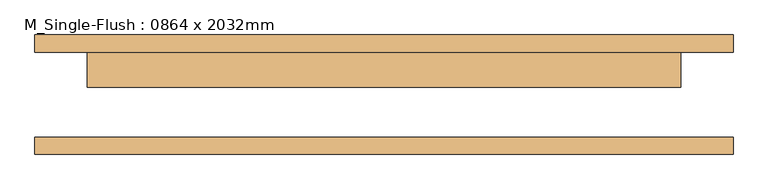
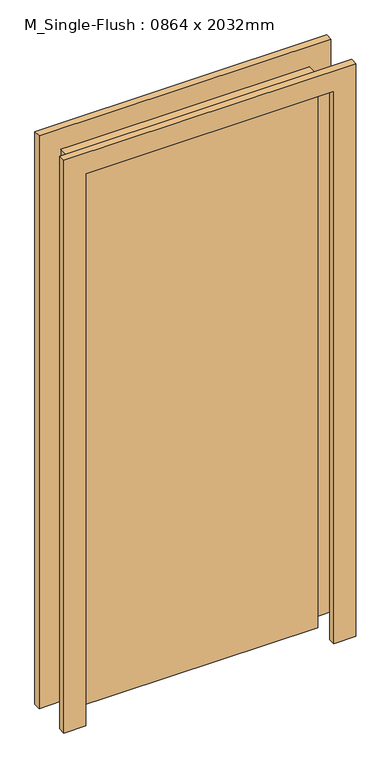
"""IFC4 building model written with IfcOpenShell, lengths in millimetres: door geometry, M_Single-Flush : 0864 x 2032mm."""

import ifcopenshell
import ifcopenshell.guid

model = None  # the IFC model being written
_history = None  # IfcOwnerHistory: only IFC2X3 demands one
_inside = {}  # id of a spatial element -> (the spatial element, [elements in it])
_under = {}  # id of a project, library or spatial element -> (it, [spatial elements below it])
_declared = {}  # id of a project -> (the project, [libraries it declares])
_typed = {}  # id of a type object -> (the type object, [elements of that type])
_made_of = {}  # id of a material, layer set ... -> (it, [elements and type objects made of it])


def new_model(schema):
    """Start an empty IFC model of exactly this schema.

    Asked for "IFC4X3", IfcOpenShell would pick the latest addendum, in which some entities
    have other attributes; the version numbers below select the first issue.
    IFC2X3 requires an IfcOwnerHistory on every rooted entity: one is made here for all.
    """
    global model, _history
    if schema == "IFC4X3":
        model = ifcopenshell.file(schema_version=(4, 3, 0, 0))
    else:
        model = ifcopenshell.file(schema=schema)
    _inside.clear()
    _under.clear()
    _declared.clear()
    _typed.clear()
    _made_of.clear()
    _history = None
    if model.schema == "IFC2X3":
        org = make("IfcOrganization", Name="unknown")
        user = make(
            "IfcPersonAndOrganization",
            ThePerson=make("IfcPerson", FamilyName="unknown"),
            TheOrganization=org,
        )
        app = make(
            "IfcApplication",
            ApplicationDeveloper=org,
            Version="unknown",
            ApplicationFullName="unknown",
            ApplicationIdentifier="unknown",
        )
        _history = make(
            "IfcOwnerHistory",
            OwningUser=user,
            OwningApplication=app,
            ChangeAction="ADDED",
            CreationDate=0,
        )
    return model


def make(cls, **values):
    """One entity of the class cls with the attributes given. An attribute that is None is left unset."""
    return model.create_entity(
        cls, **{name: value for name, value in values.items() if value is not None}
    )


def rooted(cls, **values):
    """An entity with a GlobalId (a new one), such as an element, a storey or a relation."""
    return make(cls, GlobalId=ifcopenshell.guid.new(), OwnerHistory=_history, **values)


def si_unit(unit_type, name, prefix=None):
    """IfcSIUnit, for example si_unit("LENGTHUNIT", "METRE", prefix="MILLI")."""
    return make("IfcSIUnit", UnitType=unit_type, Prefix=prefix, Name=name)


def assignment(units):
    """IfcUnitAssignment: the units of a project."""
    return None if units is None else make("IfcUnitAssignment", Units=units)


def point(xyz):
    """IfcCartesianPoint."""
    return None if xyz is None else make("IfcCartesianPoint", Coordinates=xyz)


def direction(xyz):
    """IfcDirection."""
    return None if xyz is None else make("IfcDirection", DirectionRatios=xyz)


def frame(location, z_axis=None, x_axis=None):
    """IfcAxis2Placement3D, a coordinate frame: its origin and axes. An axis left out is left unset."""
    return make(
        "IfcAxis2Placement3D",
        Location=point(location),
        Axis=direction(z_axis),
        RefDirection=direction(x_axis),
    )


def origin():
    """The frame at (0, 0, 0) with its axes left unset."""
    return frame((0.0, 0.0, 0.0))


def origin_with_axes():
    """The frame at (0, 0, 0) with the z axis (0, 0, 1) and the x axis (1, 0, 0) written out."""
    return frame((0.0, 0.0, 0.0), z_axis=(0.0, 0.0, 1.0), x_axis=(1.0, 0.0, 0.0))


def place(relative_to, where):
    """IfcLocalPlacement: puts the frame where relative to a parent placement (None: the world)."""
    return make(
        "IfcLocalPlacement", PlacementRelTo=relative_to, RelativePlacement=where
    )


def context(
    kind, dimensions, precision=None, world=None, true_north=None, identifier=None
):
    """IfcGeometricRepresentationContext, for example the 3D "Model" context."""
    return make(
        "IfcGeometricRepresentationContext",
        ContextIdentifier=identifier,
        ContextType=kind,
        CoordinateSpaceDimension=dimensions,
        Precision=precision,
        WorldCoordinateSystem=world,
        TrueNorth=true_north,
    )


def project(units=None, contexts=None):
    """IfcProject with its units and contexts."""
    return rooted(
        "IfcProject",
        Name="project",
        RepresentationContexts=contexts,
        UnitsInContext=assignment(units),
    )


def spatial(cls, under=None, at=None, **own):
    """A site, building, storey or space (cls), placed at a placement, below another one or the project."""
    s = rooted(cls, ObjectPlacement=at, **own)
    if under is not None:
        _under.setdefault(under.id(), (under, []))[1].append(s)
    return s


def polyline(points):
    """IfcPolyline through the points."""
    return make("IfcPolyline", Points=[point(p) for p in points])


def outline(outer, holes=None, kind="AREA"):
    """IfcArbitraryClosedProfileDef: a profile drawn as a closed curve; with holes, ...WithVoids."""
    if holes is None:
        return make("IfcArbitraryClosedProfileDef", ProfileType=kind, OuterCurve=outer)
    return make(
        "IfcArbitraryProfileDefWithVoids",
        ProfileType=kind,
        OuterCurve=outer,
        InnerCurves=holes,
    )


def extrude(swept, where, along, depth):
    """IfcExtrudedAreaSolid: the profile swept, set in the frame where, extruded along a direction by depth."""
    return make(
        "IfcExtrudedAreaSolid",
        SweptArea=swept,
        Position=where,
        ExtrudedDirection=direction(along),
        Depth=depth,
    )


def shape(context_of_items, identifier, shape_type, items):
    """IfcShapeRepresentation: the items that make up one representation, for example the "Body"."""
    return make(
        "IfcShapeRepresentation",
        ContextOfItems=context_of_items,
        RepresentationIdentifier=identifier,
        RepresentationType=shape_type,
        Items=items,
    )


def source(mapping_origin, context_of_items, identifier, shape_type, items):
    """IfcRepresentationMap: a shape defined once, which mapped items show again and again."""
    return make(
        "IfcRepresentationMap",
        MappingOrigin=mapping_origin,
        MappedRepresentation=shape(context_of_items, identifier, shape_type, items),
    )


def transform(
    local_origin,
    x_axis=None,
    y_axis=None,
    z_axis=None,
    scale=None,
    scale2=None,
    scale3=None,
    uniform=True,
):
    """IfcCartesianTransformationOperator3D, or its non-uniform kind. x_axis, y_axis, z_axis: its Axis1, 2, 3."""
    if uniform:
        return make(
            "IfcCartesianTransformationOperator3D",
            Axis1=direction(x_axis),
            Axis2=direction(y_axis),
            LocalOrigin=point(local_origin),
            Scale=scale,
            Axis3=direction(z_axis),
        )
    return make(
        "IfcCartesianTransformationOperator3DnonUniform",
        Axis1=direction(x_axis),
        Axis2=direction(y_axis),
        LocalOrigin=point(local_origin),
        Scale=scale,
        Axis3=direction(z_axis),
        Scale2=scale2,
        Scale3=scale3,
    )


def mapped(mapping_source, mapping_target):
    """IfcMappedItem: shows the shape of a source again, moved by a transform."""
    return make(
        "IfcMappedItem", MappingSource=mapping_source, MappingTarget=mapping_target
    )


def made_of(thing, what):
    """Note that an element or type object is made of a material, layer set ...; save() writes the relation."""
    if what is not None:
        _made_of.setdefault(what.id(), (what, []))[1].append(thing)
    return thing


def element(
    cls,
    number,
    at=None,
    inside=None,
    cuts=None,
    type_object=None,
    material=None,
    context=None,
    identifier="Body",
    shape_type=None,
    held_by="IfcProductDefinitionShape",
    body=None,
    shapes=None,
    **own,
):
    """One element of the class cls, such as IfcWall. Its Tag is "e" and its number.

    at: its placement. inside: the storey or other place that contains it. cuts: it is an
    opening in that element (IfcRelVoidsElement). A single representation is given by context,
    identifier, shape_type and body (its items); several are given by shapes. held_by: the class
    of the entity that holds the representations. save() writes the other relations.
    """
    e = rooted(cls, Tag="e%d" % number, ObjectPlacement=at, **own)
    if body is not None:
        shapes = [shape(context, identifier, shape_type, body)]
    if shapes is not None:
        e.Representation = make(held_by, Representations=shapes)
    if inside is not None:
        _inside.setdefault(inside.id(), (inside, []))[1].append(e)
    if cuts is not None:
        rooted(
            "IfcRelVoidsElement", RelatingBuildingElement=cuts, RelatedOpeningElement=e
        )
    if type_object is not None:
        _typed.setdefault(type_object.id(), (type_object, []))[1].append(e)
    return made_of(e, material)


def aggregate(whole, parts):
    """IfcRelAggregates: a whole, such as a stair, and the parts it consists of."""
    return rooted("IfcRelAggregates", RelatingObject=whole, RelatedObjects=parts)


def save(model, path):
    """Write the relations noted so far, then the file.

    IfcRelAggregates (storeys below a building ...), IfcRelContainedInSpatialStructure (elements
    in a storey), IfcRelDefinesByType, IfcRelAssociatesMaterial and IfcRelDeclares: one each for
    every whole, place, type object, material and project.
    """
    for whole, parts in _under.values():
        aggregate(whole, parts)
    for where, things in _inside.values():
        rooted(
            "IfcRelContainedInSpatialStructure",
            RelatedElements=things,
            RelatingStructure=where,
        )
    for kind, things in _typed.values():
        rooted("IfcRelDefinesByType", RelatedObjects=things, RelatingType=kind)
    for what, things in _made_of.values():
        rooted("IfcRelAssociatesMaterial", RelatedObjects=things, RelatingMaterial=what)
    for by, libraries in _declared.values():
        rooted("IfcRelDeclares", RelatingContext=by, RelatedDefinitions=libraries)
    model.write(path)


def m_single_flush_0864_x_2032mm_f1a57c69(model_context):
    return source(origin(), model_context, "Body", "SweptSolid", [
        extrude(outline(polyline([(2108.0, -508.0), (0.0, -508.0), (0.0, -432.0), (2032.0, -432.0), (2032.0, 432.0), (0.0, 432.0), (0.0, 508.0), (2108.0, 508.0), (2108.0, -508.0)])), frame((0.0, 62.0, 0.0), z_axis=(0.0, 1.0, 0.0), x_axis=(0.0, 0.0, 1.0)), (0.0, 0.0, 1.0), 25.0),
        extrude(outline(polyline([(2108.0, 508.0), (2108.0, -508.0), (0.0, -508.0), (0.0, -432.0), (2032.0, -432.0), (2032.0, 432.0), (0.0, 432.0), (0.0, 508.0), (2108.0, 508.0)])), frame((0.0, -87.0, 0.0), z_axis=(0.0, 1.0, 0.0), x_axis=(0.0, 0.0, 1.0)), (0.0, 0.0, 1.0), 25.0),
        extrude(outline(polyline([(432.0, 11.0), (-432.0, 11.0), (-432.0, 62.0), (432.0, 62.0), (432.0, 11.0)])), origin_with_axes(), (0.0, 0.0, 1.0), 2032.0),
    ])


if __name__ == "__main__":
    model = new_model("IFC4")
    model_context = context("Model", 3, world=origin())
    ifc_project = project(units=[si_unit("LENGTHUNIT", "METRE", prefix="MILLI")], contexts=[model_context])
    site = spatial("IfcSite", under=ifc_project)
    building = spatial("IfcBuilding", under=site)
    placement = place(None, origin())
    m_single_flush_0864_x_2032mm_shape = m_single_flush_0864_x_2032mm_f1a57c69(model_context)
    element("IfcDoor", 1, ObjectType="M_Single-Flush : 0864 x 2032mm", at=placement, inside=building, context=model_context, shape_type="MappedRepresentation", body=[
        mapped(m_single_flush_0864_x_2032mm_shape, transform((0.0, 0.0, 0.0), x_axis=(1.0, 0.0, 0.0), y_axis=(0.0, 1.0, 0.0), z_axis=(0.0, 0.0, 1.0))),
    ])
    save(model, "model.ifc")

# Revit data of these elements
# Type "M_Single-Flush : 0864 x 2032mm"
#   Manufacturer = "Manufacturer"
#   Type Mark = "32"
#   Construction Type = "Construction Type"
#   Fire Rating = "Fire Rating"
#   AccessibilityPerformance = "AccessibilityPerformance"
#   CodePerformance = "CodePerformance"
#   IsFireExit = "IsFireExit"
#   ConstructionType = "ConstructionType"
#   GlazingAreaFraction = "GlazingAreaFraction"
#   OperationType = "OperationType"
#   Area = "Area"
#   Color = "Color"
#   Constituents = "Constituents"
#   Features = "Features"
#   Finish = "Finish"
#   Grade = "Grade"
#   Material = "Material"
#   ModelReference = "ModelReference"
#   NominalHeight = "NominalHeight"
#   NominalLength = "NominalLength"
#   NominalWidth = "NominalWidth"
#   ProductionYear = "ProductionYear"
#   Reference = "Reference"
#   Shape = "Shape"
#   Size = "Size"
#   SustainabilityPerformance = "SustainabilityPerformance"
#   WarrantyDescription = "WarrantyDescription"
#   WarrantyDurationLabor = "WarrantyDurationLabor"
#   WarrantyDurationParts = "WarrantyDurationParts"
#   WarrantyGuarantorLabor = "WarrantyGuarantorLabor"
#   WarrantyGuarantorParts = "WarrantyGuarantorParts"
#   ExpectedLife = "ExpectedLife"
#   ReplacementCost = "ReplacementCost"
#   AssetAccountingType = "FIXED"
#   ModelLabel = "ModelLabel"
#   Thickness = 0.051 m
#   Height = 2.032 m
#   Trim Projection Ext = 0.025 m
#   Trim Projection Int = 0.025 m
#   Trim Width = 0.076 m
#   Width = 0.864 m
#   Door Material = Door - Panel
#   Frame Material = Door - Frame
#   Function = (empty or 0)
#   Wall Closure = (empty or 0)
# Element 1 (IfcDoor, "M_Single-Flush : 0864 x 2032mm")
#   Materials on its faces: "Door - Frame", "Door - Panel"
# Materials
#   "Door - Panel": class "Wood", colour RGB 210 159 95, transparency 0
#   "Door - Frame": class "Miscellaneous", colour RGB 118 70 51, transparency 0
